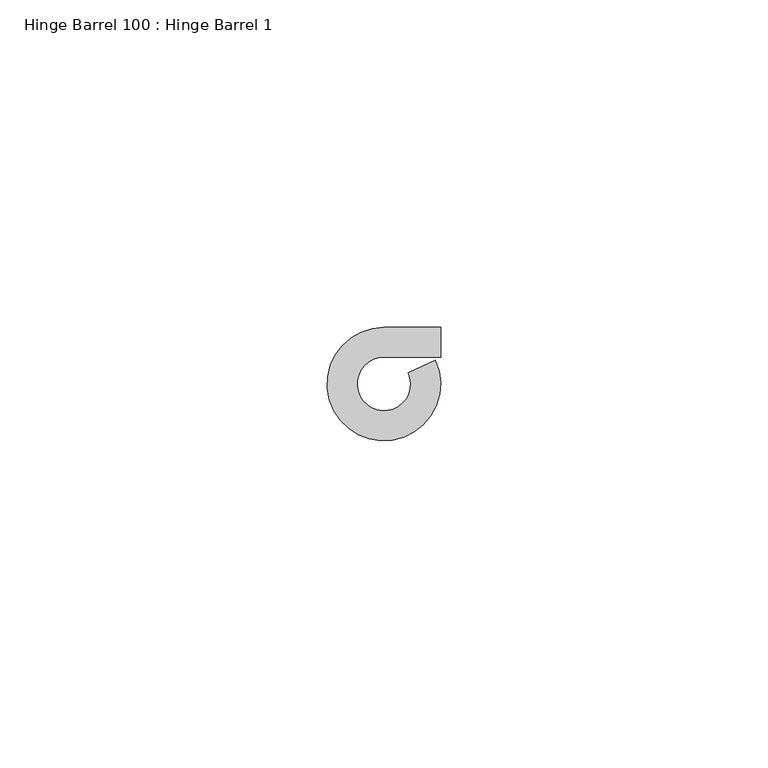
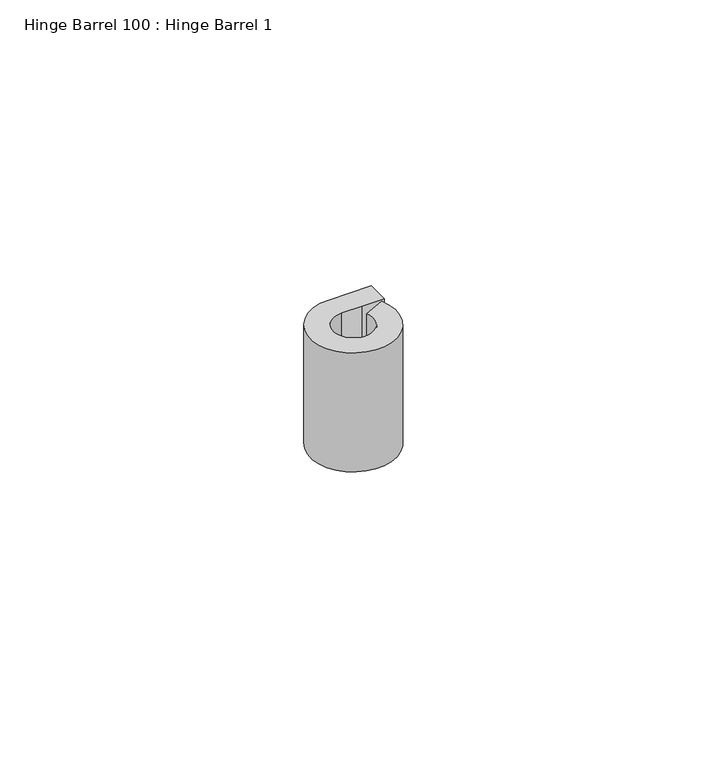
"""IFC4 building model written with IfcOpenShell, lengths in millimetres: proxy geometry, Hinge Barrel 100 : Hinge Barrel 1."""

from ifc_helpers import new_model, si_unit, point, frame, frame_2d, origin, place, context, project, spatial, polyline, circle_curve, trimmed, segment, composite_curve, outline, extrude, source, transform, mapped, element, save


def hinge_barrel_100_hinge_barrel_1_43aeb578(model_context):
    return source(origin(), model_context, "Body", "SweptSolid", [
        extrude(outline(composite_curve([segment(polyline([(587323.2214739, -533980.5883841), (587319.1320739, -533980.5883841)]), True, "CONTINUOUS"), segment(trimmed(circle_curve(frame_2d((587319.1320739, -533984.6777841)), 4.0894), [point((587319.1320739, -533980.5883841))], [point((587322.8436736, -533982.9610371))], True, "CARTESIAN"), True, "CONTINUOUS"), segment(polyline([(587322.8436736, -533982.9610371), (587326.986084, -533981.0450249)]), True, "CONTINUOUS"), segment(trimmed(circle_curve(frame_2d((587319.1320739, -533984.6777841)), 8.6534625), [point((587326.986084, -533981.0450249))], [point((587319.1320739, -533976.0243216))], False, "CARTESIAN"), True, "CONTINUOUS"), segment(polyline([(587319.1320739, -533976.0243216), (587327.7934739, -533976.0243216), (587327.7934739, -533980.5883841), (587323.2214739, -533980.5883841)]), True, "CONTINUOUS")], self_intersect=False)), frame((0.0, 0.0, 2038.35), z_axis=(0.0, 0.0, 1.0), x_axis=(1.0, 0.0, 0.0)), (0.0, 0.0, 1.0), 25.4),
    ])


if __name__ == "__main__":
    model = new_model("IFC4")
    model_context = context("Model", 3, world=origin())
    ifc_project = project(units=[si_unit("LENGTHUNIT", "METRE", prefix="MILLI")], contexts=[model_context])
    site = spatial("IfcSite", under=ifc_project)
    building = spatial("IfcBuilding", under=site)
    placement = place(None, origin())
    hinge_barrel_100_hinge_barrel_1_shape = hinge_barrel_100_hinge_barrel_1_43aeb578(model_context)
    element("IfcBuildingElementProxy", 1, Name="Hinge Barrel 100 : Hinge Barrel 1", ObjectType="Hinge Barrel 100 : Hinge Barrel 1", at=placement, inside=building, context=model_context, shape_type="MappedRepresentation", body=[
        mapped(hinge_barrel_100_hinge_barrel_1_shape, transform((0.0, 0.0, 0.0), x_axis=(1.0, 0.0, 0.0), y_axis=(0.0, 1.0, 0.0), z_axis=(0.0, 0.0, 1.0))),
    ])
    save(model, "model.ifc")

# Revit data of these elements
# Element 1 (IfcBuildingElementProxy, "Hinge Barrel 100 : Hinge Barrel 1")
#   Materials on its faces: "6\"X6\" WELD-ON STL BUTT HINGE"
# Materials
#   "6\"X6\" WELD-ON STL BUTT HINGE": class "Metal", colour RGB 189 187 185, transparency 0, Description = "Carbon steel", Cost = 0
